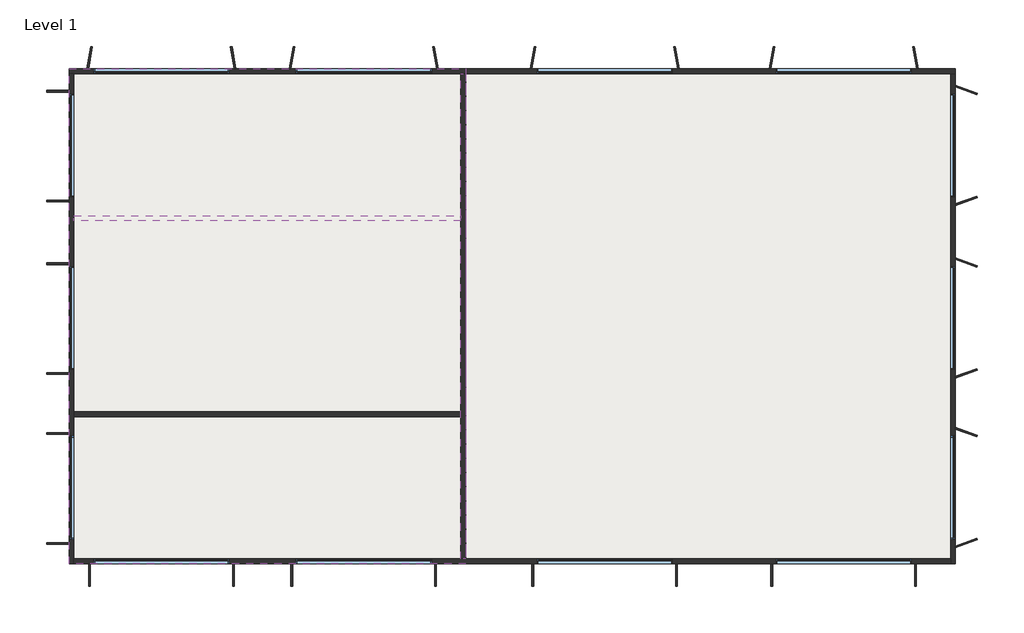
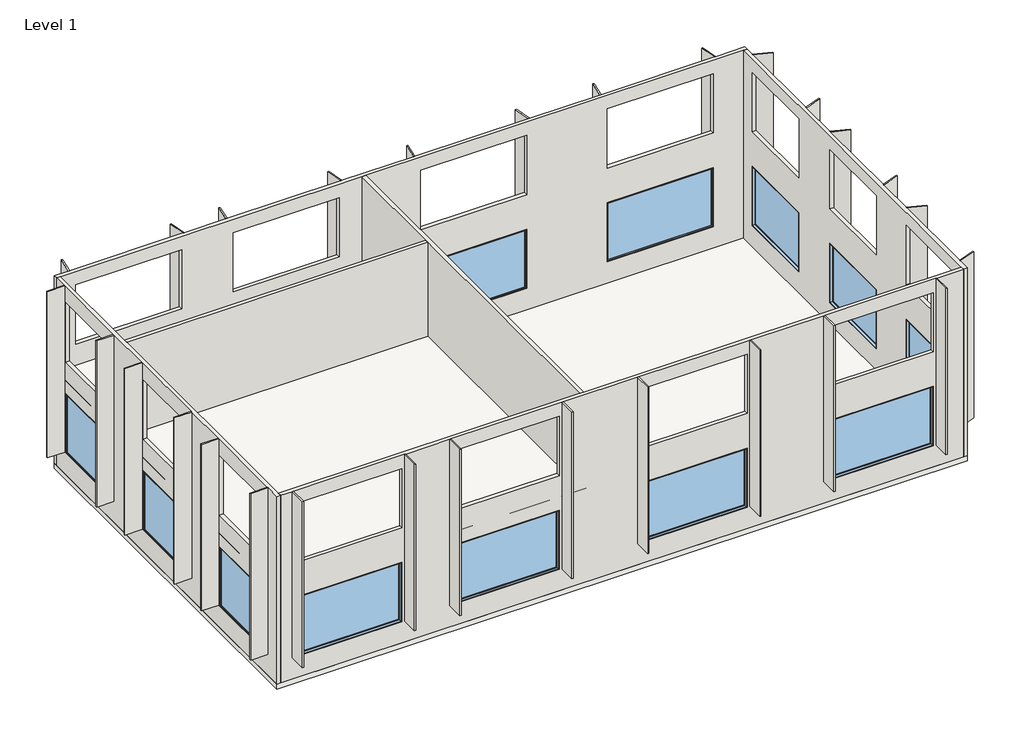
# One storey: 36 walls, 14 windows, 2 slabs.
# Revit data of these elements (continued)
# Type "M_Fixed : 2500x 3220mm" (continued)
#   Type Mark = "26"
#   Height = 2500 mm
#   Default Sill Height = 305 mm
#   Width = 3219.6 mm
#   Window Inset = 19 mm
#   Frame Exterior Material = Sash
#   Frame Interior Material = Sash
#   Glass Pane Material = Glass
#   Sash = Sash
#   Wall Closure = (empty or 0)
# Element 1 (IfcSlab, "160mm Concrete With 50mm Metal Deck")
#   Height Offset From Level = 0 mm
#   Phase Created = New Construction
#   Materials on its faces: "Metal Deck", "Default Floor"
# Element 2 (IfcSlab, "160mm Concrete With 50mm Metal Deck")
#   Height Offset From Level = 3962.4 mm
#   Phase Created = New Construction
#   Materials on its faces: "Metal Deck", "Default Floor"
# Elements 3, 4, 5, 6 (IfcWall, "Generic - 152.4mm")
#   Top Offset = 0 mm
#   Base Offset = 0 mm
#   wall height = 7924.8 mm
#   Phase Created = New Construction
#   Base Constraint = Level 1
#   Top Constraint = Roof Level
#   Materials on its faces: "Default Wall"
# Element 7 (IfcWall, "Generic - 152.4mm - Interior")
#   Top Offset = 3962.4 mm
#   Base Offset = 0 mm
#   wall height = 3752.4 mm
#   Phase Created = New Construction
#   Base Constraint = Level 1
#   Top Constraint = Level 1
#   Materials on its faces: "Default Wall"
# Element 8 (IfcWall, "Generic - 152.4mm - Interior")
#   Top Offset = 3862.4 mm
#   Base Offset = 0 mm
#   wall height = 3752.4 mm
#   Phase Created = New Construction
#   Base Constraint = Level 1
#   Top Constraint = Level 1
#   Materials on its faces: "Default Wall"
# Elements 9, 10 (IfcWall, "Generic - 152.4mm - Interior")
#   built-in parameter 1001111 = 3962.4 mm
#   Top Offset = 0 mm
#   Base Offset = 3962.4 mm
#   Unconnected Height = 3962.4 mm
#   wall height = 3962.4 mm
#   Phase Created = New Construction
#   Base Constraint = Level 1
#   Top Constraint = Roof Level
#   Materials on its faces: "Default Wall"
# Elements 11, 12, 13, 14, 15, 16, 17, 18, 19, 20, 21, 22, 23, 24, 25, 26, 27, 28, 29, 30, 31, 32, 33, 34, 35, 36, 37, 38 (IfcWall, "Shading devices")
#   built-in parameter 1001111 = 902.4 mm
#   Top Offset = 0 mm
#   Base Offset = 902.4 mm
#   wall height = 7022.4 mm
#   Phase Created = New Construction
#   Base Constraint = Level 1
#   Top Constraint = Roof Level
#   Materials on its faces: "Default Wall"
# Element 39 (IfcWindow, "M_Fixed : 2500X 4228mm")
#   Mark = "10"
#   Phase Created = New Construction
#   Materials on its faces: "Sash", "Glass"
# Element 40 (IfcWindow, "M_Fixed : 2500X 4228mm")
#   Mark = "11"
#   Phase Created = New Construction
#   Materials on its faces: "Sash", "Glass"
# Element 41 (IfcWindow, "M_Fixed : 2500X 4228mm")
#   Mark = "12"
#   Phase Created = New Construction
#   Materials on its faces: "Sash", "Glass"
# Element 42 (IfcWindow, "M_Fixed : 2500X 4228mm")
#   Mark = "13"
#   Phase Created = New Construction
#   Materials on its faces: "Sash", "Glass"
# Element 43 (IfcWindow, "M_Fixed : 2500X 4228mm")
#   Mark = "14"
#   Phase Created = New Construction
#   Materials on its faces: "Sash", "Glass"
# Element 44 (IfcWindow, "M_Fixed : 2500X 4228mm")
#   Mark = "15"
#   Phase Created = New Construction
#   Materials on its faces: "Sash", "Glass"
# Element 45 (IfcWindow, "M_Fixed : 2500X 4228mm")
#   Mark = "16"
#   Phase Created = New Construction
#   Materials on its faces: "Sash", "Glass"
# Element 46 (IfcWindow, "M_Fixed : 2500X 4228mm")
#   Mark = "17"
#   Phase Created = New Construction
#   Materials on its faces: "Sash", "Glass"
# Element 47 (IfcWindow, "M_Fixed : 2500x 3220mm")
#   Mark = "26"
#   Phase Created = New Construction
#   Materials on its faces: "Sash", "Glass"
# Element 48 (IfcWindow, "M_Fixed : 2500x 3220mm")
#   Mark = "28"
#   Phase Created = New Construction
#   Materials on its faces: "Sash", "Glass"
# Element 49 (IfcWindow, "M_Fixed : 2500x 3220mm")
#   Mark = "29"
#   Phase Created = New Construction
#   Materials on its faces: "Sash", "Glass"
# Element 50 (IfcWindow, "M_Fixed : 2500x 3220mm")
#   Mark = "30"
#   Phase Created = New Construction
#   Materials on its faces: "Sash", "Glass"
# Element 51 (IfcWindow, "M_Fixed : 2500x 3220mm")
#   Mark = "31"
#   Phase Created = New Construction
#   Materials on its faces: "Sash", "Glass"
# Element 52 (IfcWindow, "M_Fixed : 2500x 3220mm")
#   Mark = "32"
#   Phase Created = New Construction
#   Materials on its faces: "Sash", "Glass"
# Materials
#   "Metal Deck": class "Metal", colour RGB 247 247 247, transparency 0, Description = "Steel, mill finish", Cost = 0
#   "Sash": class "Wood", colour RGB 136 99 55, transparency 0
#   "Glass": class "Glass", colour RGB 0 128 192, transparency 0.9, Description = "Soda Lime Glass", Cost = 0
#   "Default Floor": class "Miscellaneous", colour RGB 127 127 127, transparency 0, Cost = 0
#   "Default Wall": class "Miscellaneous", colour RGB 128 128 128, transparency 0, Cost = 0
# Room at (7259.725, -1600.456) mm, phase "New Construction", upper level "Level 2", upper offset 0 mm, lower offset 0 mm
#   Number = "6"
#   Name = "Room"
# Room at (8198.725, 4816.984) mm, phase "New Construction", upper level "Level 2", upper offset 0 mm, lower offset 0 mm
#   Number = "7"
#   Name = "Room"
# Room at (21274.823, 2677.837) mm, phase "New Construction", upper level "Roof Level", upper offset 0 mm, lower offset 0 mm
#   Number = "8"
#   Name = "Room"
